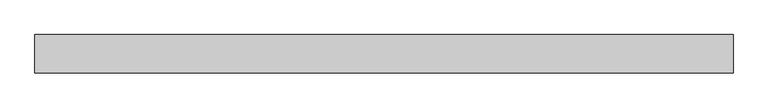
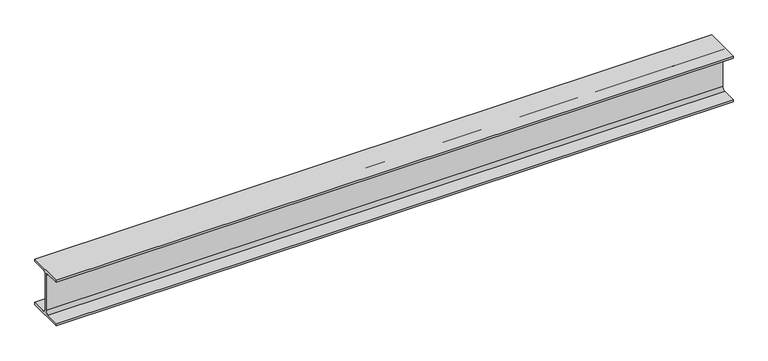
"""IFC4 building model written with IfcOpenShell, lengths in millimetres: beam geometry, 0912_Steel Framing_H-KSD3502 : H_SB_ASB_H-194x150x6x9."""

from ifc_helpers import new_model, si_unit, point, frame, frame_2d, origin, place, context, project, spatial, polyline, circle_curve, trimmed, segment, composite_curve, outline, extrude, source, transform, mapped, element, save


def beam_c4fcb7a9(model_context):
    return source(origin(), model_context, "Body", "SweptSolid", [
        extrude(outline(composite_curve([segment(polyline([(75.0, -88.0), (75.0, -97.0), (-75.0, -97.0), (-75.0, -88.0), (-16.0, -88.0)]), True, "CONTINUOUS"), segment(trimmed(circle_curve(frame_2d((-16.0, -75.0)), 13.0), [point((-16.0, -88.0))], [point((-3.0, -75.0))], True, "CARTESIAN"), True, "CONTINUOUS"), segment(polyline([(-3.0, -75.0), (-3.0, 75.0)]), True, "CONTINUOUS"), segment(trimmed(circle_curve(frame_2d((-16.0, 75.0)), 13.0), [point((-3.0, 75.0))], [point((-16.0, 88.0))], True, "CARTESIAN"), True, "CONTINUOUS"), segment(polyline([(-16.0, 88.0), (-75.0, 88.0), (-75.0, 97.0), (75.0, 97.0), (75.0, 88.0), (16.0, 88.0)]), True, "CONTINUOUS"), segment(trimmed(circle_curve(frame_2d((16.0, 75.0)), 13.0), [point((16.0, 88.0))], [point((3.0, 75.0))], True, "CARTESIAN"), True, "CONTINUOUS"), segment(polyline([(3.0, 75.0), (3.0, -75.0)]), True, "CONTINUOUS"), segment(trimmed(circle_curve(frame_2d((16.0, -75.0)), 13.0), [point((3.0, -75.0))], [point((16.0, -88.0))], True, "CARTESIAN"), True, "CONTINUOUS"), segment(polyline([(16.0, -88.0), (75.0, -88.0)]), True, "CONTINUOUS")], self_intersect=False)), frame((-1236.0559406, 0.0, 0.0), z_axis=(1.0, 0.0, 0.0), x_axis=(0.0, 1.0, 0.0)), (0.0, 0.0, 1.0), 2729.2385396),
    ])


if __name__ == "__main__":
    model = new_model("IFC4")
    model_context = context("Model", 3, world=origin())
    ifc_project = project(units=[si_unit("LENGTHUNIT", "METRE", prefix="MILLI")], contexts=[model_context])
    site = spatial("IfcSite", under=ifc_project)
    building = spatial("IfcBuilding", under=site)
    placement = place(None, origin())
    beam_shape = beam_c4fcb7a9(model_context)
    element("IfcBeam", 1, ObjectType="0912_Steel Framing_H-KSD3502 : H_SB_ASB_H-194x150x6x9", at=placement, inside=building, context=model_context, shape_type="MappedRepresentation", body=[
        mapped(beam_shape, transform((0.0, 0.0, 0.0), x_axis=(1.0, 0.0, 0.0), y_axis=(0.0, 1.0, 0.0), z_axis=(0.0, 0.0, 1.0))),
    ])
    save(model, "model.ifc")

# Revit data of these elements
# Type "0912_Steel Framing_H-KSD3502 : H_SB_ASB_H-194x150x6x9"
#   H_WM Code_1 = "S01AA002-00001 | Main Steel Structure Fabrication Work | Shelter/Building | Medium Steel - Standard (90KG/M>Weight≥30KG/M) | Material: (   )"
#   H_WM Code_2 = "S03AA028-00001 | Main Steel Structure Erection Work | Shelter/Building | Medium Steel (90KG/M>Weight≥30KG/M) | Material: (   )"
#   H_WM Code_3 = "S01AA010-00001 | Main Steel Structure Fabrication Work | Shelter/Building | Steel Painting/Coating | for Non-Fireproofed Steel Surface, Surface Preparation, Primer, Second & Final Coat | Material: (   )"
#   H_Q'ty Cal Type Tag = "SB-Q2"
#   Width = 15.0 cm
#   Web Thickness = 0.6 cm
#   Web Fillet = 1.3 cm
#   Warping Constant = 43316.0 cm⁶
#   W = 0
#   Torsional Moment of Inertia = 8.622 cm⁴
#   Section Area = 39.01 cm²
#   Plastic Modulus weak axis = 104.0 cm³
#   Plastic Modulus strong axis = 309.0 cm³
#   Perimeter = 0.95 m²/m
#   Nominal Weight = 30.60 kgf/m
#   Moment of Inertia weak axis = 507.00 cm⁴
#   Moment of Inertia strong axis = 2690.00 cm⁴
#   Height = 19.4 cm
#   Flange Thickness = 0.9 cm
#   Elastic Modulus weak axis = 67.6 cm³
#   Elastic Modulus strong axis = 277.0 cm³
#   Centroid Vertical = 9.7 cm
#   Centroid Horizontal = 7.5 cm
#   Ix = 26900000
#   Length [instance default] = 1.5240 m
#   Zx = 309000
#   b = 0.1500 m
#   h = 0.1940 m
#   r = 0.0130 m
#   s = 0.0060 m
#   t = 0.0090 m
#   A = 0.003901 m²
#   Structural Material [instance default] = Steel, 45-345
#   Assembly Code = ""
# Element 1 (IfcBeam, "0912_Steel Framing_H-KSD3502 : H_SB_ASB_H-194x150x6x9")
#   Structural Material = none
# Materials
#   "Steel, 45-345": class "Metal", colour RGB 189 187 185, transparency 0, Description = "Steel 345 MPa", Cost = 0
